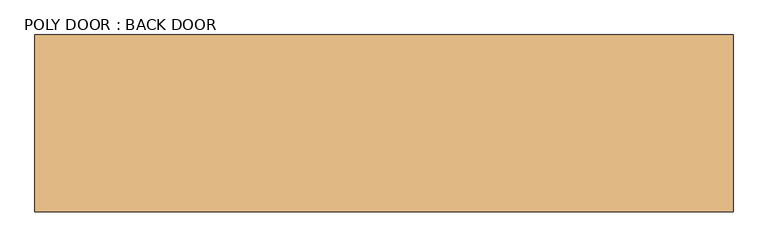
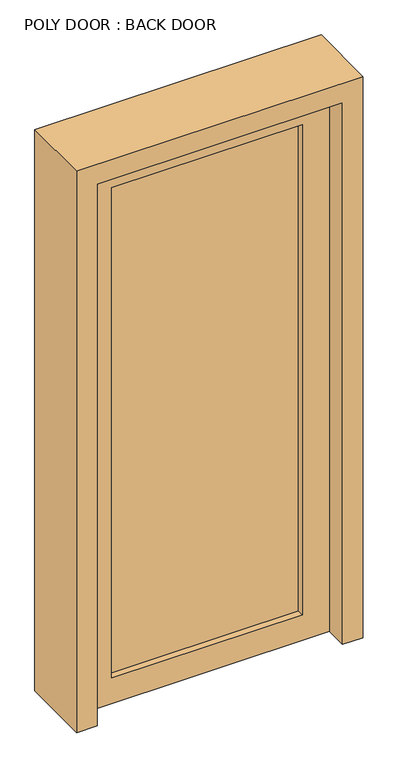
"""IFC4 building model written with IfcOpenShell, lengths in millimetres: door geometry, POLY DOOR : BACK DOOR."""

from ifc_helpers import new_model, si_unit, frame, origin, place, context, project, spatial, polyline, outline, extrude, source, transform, mapped, element, save


def poly_door_back_door_c4b8b8a1(model_context):
    return source(origin(), model_context, "Body", "SweptSolid", [
        extrude(outline(polyline([(355.6, -25.4), (-355.6, -25.4), (-355.6, -12.7), (355.6, -12.7), (355.6, -25.4)])), frame((0.0, 0.0, 101.6), z_axis=(0.0, 0.0, 1.0), x_axis=(1.0, 0.0, 0.0)), (0.0, 0.0, 1.0), 1930.4),
        extrude(outline(polyline([(2133.6, 457.2), (2133.6, -457.2), (0.0, -457.2), (0.0, 457.2), (2133.6, 457.2)]), holes=[polyline([(2032.0, 355.6), (101.6, 355.6), (101.6, -355.6), (2032.0, -355.6), (2032.0, 355.6)])]), frame((0.0, -50.8, 0.0), z_axis=(0.0, 1.0, 0.0), x_axis=(0.0, 0.0, 1.0)), (0.0, 0.0, 1.0), 50.8),
        extrude(outline(polyline([(2209.8, -533.4), (0.0, -533.4), (0.0, -457.2), (2133.6, -457.2), (2133.6, 457.2), (0.0, 457.2), (0.0, 533.4), (2209.8, 533.4), (2209.8, -533.4)])), frame((0.0, -134.9375, 0.0), z_axis=(0.0, 1.0, 0.0), x_axis=(0.0, 0.0, 1.0)), (0.0, 0.0, 1.0), 269.875),
    ])


if __name__ == "__main__":
    model = new_model("IFC4")
    model_context = context("Model", 3, world=origin())
    ifc_project = project(units=[si_unit("LENGTHUNIT", "METRE", prefix="MILLI")], contexts=[model_context])
    site = spatial("IfcSite", under=ifc_project)
    building = spatial("IfcBuilding", under=site)
    placement = place(None, origin())
    poly_door_back_door_shape = poly_door_back_door_c4b8b8a1(model_context)
    element("IfcDoor", 1, ObjectType="POLY DOOR : BACK DOOR", at=placement, inside=building, context=model_context, shape_type="MappedRepresentation", body=[
        mapped(poly_door_back_door_shape, transform((0.0, 0.0, 0.0), x_axis=(1.0, 0.0, 0.0), y_axis=(0.0, 1.0, 0.0), z_axis=(0.0, 0.0, 1.0))),
    ])
    save(model, "model.ifc")

# Revit data of these elements
# Type "POLY DOOR : BACK DOOR"
#   Type Mark = "64"
#   Assembly Code = "C1020"
#   Analytic Construction = "<None>"
#   Thickness = 0' - 2"
#   Glass Inset = 0' - 4"
#   Height = 7' - 0"
#   Trim Projection Ext = 0' - 1"
#   Trim Projection Int = 0' - 1"
#   Trim Width = 0' - 3"
#   Width = 3' - 0"
#   WINDOW = yes
#   Glass Material = INSULATED GLAZING
#   Door Material = ALUMINUM STOREFRONT
#   Frame Material = ALUMINUM STOREFRONT
#   Function = (empty or 0)
#   Wall Closure = (empty or 0)
# Element 1 (IfcDoor, "POLY DOOR : BACK DOOR")
#   Materials on its faces: "ALUMINUM STOREFRONT", "INSULATED GLAZING"
# Materials
#   "INSULATED GLAZING": class "Glass", colour RGB 196 205 210, transparency 0.85, Description = "Soda Lime Glass", Cost = 0
#   "ALUMINUM STOREFRONT": class "Metal", colour RGB 244 244 244, transparency 0, Description = "Aluminum 6061", Cost = 0
